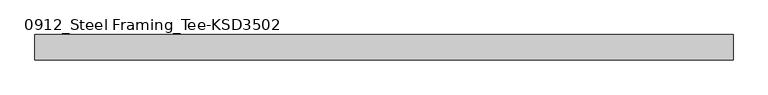
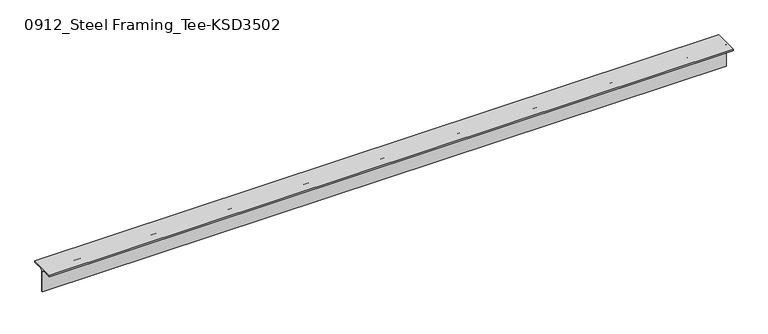
"""IFC4 building model written with IfcOpenShell, lengths in millimetres: member geometry, 0912_Steel Framing_Tee-KSD3502 : H_SB_ASB_CT-150x150x6.5x9."""

from ifc_helpers import new_model, si_unit, point, frame, frame_2d, origin, place, context, project, spatial, polyline, circle_curve, trimmed, segment, composite_curve, outline, extrude, source, transform, mapped, element, save


def member_0912_steel_framing_tee_ksd3502_b108f944(model_context):
    return source(origin(), model_context, "Body", "SweptSolid", [
        extrude(outline(composite_curve([segment(polyline([(-75.0, 75.0), (75.0, 75.0), (75.0, 66.0), (16.25, 66.0)]), True, "CONTINUOUS"), segment(trimmed(circle_curve(frame_2d((16.25, 53.0)), 13.0), [point((16.25, 66.0))], [point((3.25, 53.0))], True, "CARTESIAN"), True, "CONTINUOUS"), segment(polyline([(3.25, 53.0), (3.25, -75.0), (-3.25, -75.0), (-3.25, 53.0)]), True, "CONTINUOUS"), segment(trimmed(circle_curve(frame_2d((-16.25, 53.0)), 13.0), [point((-3.25, 53.0))], [point((-16.25, 66.0))], True, "CARTESIAN"), True, "CONTINUOUS"), segment(polyline([(-16.25, 66.0), (-75.0, 66.0), (-75.0, 75.0)]), True, "CONTINUOUS")], self_intersect=False)), frame((-2046.1, 0.0, 0.0), z_axis=(1.0, 0.0, 0.0), x_axis=(0.0, 1.0, 0.0)), (0.0, 0.0, 1.0), 4105.6),
    ])


if __name__ == "__main__":
    model = new_model("IFC4")
    model_context = context("Model", 3, world=origin())
    ifc_project = project(units=[si_unit("LENGTHUNIT", "METRE", prefix="MILLI")], contexts=[model_context])
    site = spatial("IfcSite", under=ifc_project)
    building = spatial("IfcBuilding", under=site)
    placement = place(None, origin())
    member_0912_steel_framing_tee_ksd3502_shape = member_0912_steel_framing_tee_ksd3502_b108f944(model_context)
    element("IfcMember", 1, ObjectType="0912_Steel Framing_Tee-KSD3502 : H_SB_ASB_CT-150x150x6.5x9", at=placement, inside=building, context=model_context, shape_type="MappedRepresentation", body=[
        mapped(member_0912_steel_framing_tee_ksd3502_shape, transform((0.0, 0.0, 0.0), x_axis=(1.0, 0.0, 0.0), y_axis=(0.0, 1.0, 0.0), z_axis=(0.0, 0.0, 1.0))),
    ])
    save(model, "model.ifc")

# Revit data of these elements
# Type "0912_Steel Framing_Tee-KSD3502 : H_SB_ASB_CT-150x150x6.5x9"
#   H_WM Code_1 = "S01AA003-00001 | Main Steel Structure Fabrication Work | Shelter/Building | Light Steel - Standard (30KG/M>Weight) | Material: (   )"
#   H_WM Code_2 = "S03AA029-00001 | Main Steel Structure Erection Work | Shelter/Building | Light Steel (30KG/M>Weight) | Material: (   )"
#   H_WM Code_3 = "S01AA010-00001 | Main Steel Structure Fabrication Work | Shelter/Building | Steel Painting/Coating | for Non-Fireproofed Steel Surface, Surface Preparation, Primer, Second & Final Coat | Material: (   )"
#   H_Q'ty Cal Type Tag = "SB-Q2"
#   Width = 15.0 cm
#   Web Thickness = 0.65 cm
#   Web Fillet = 1.3 cm
#   Section Area = 23.39 cm²
#   Perimeter = 0.60 m²/m
#   Nominal Weight = 18.40 kgf/m
#   Height = 15.0 cm
#   Flange Thickness = 0.9 cm
#   Centroid Vertical = 7.5 cm
#   Centroid Horizontal = 7.5 cm
#   Length [instance default] = 1.5000 m
#   Structural Material [instance default] = Steel, 45-345
#   Warping Constant = (empty or 0)
#   Torsional Moment of Inertia = 0
#   Section Name Key = ""
#   Plastic Modulus weak axis = 0
#   Plastic Modulus strong axis = 0
#   Moment of Inertia weak axis = 0
#   Moment of Inertia strong axis = 0
#   Elastic Modulus weak axis = 0
#   Elastic Modulus strong axis = 0
#   Bolt Spacing = 0
#   Assembly Code = ""
# Element 1 (IfcMember, "0912_Steel Framing_Tee-KSD3502 : H_SB_ASB_CT-150x150x6.5x9")
#   Structural Material = none
# Materials
#   "Steel, 45-345": class "Metal", colour RGB 189 187 185, transparency 0, Description = "Steel 345 MPa", Cost = 0
